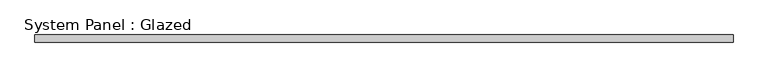
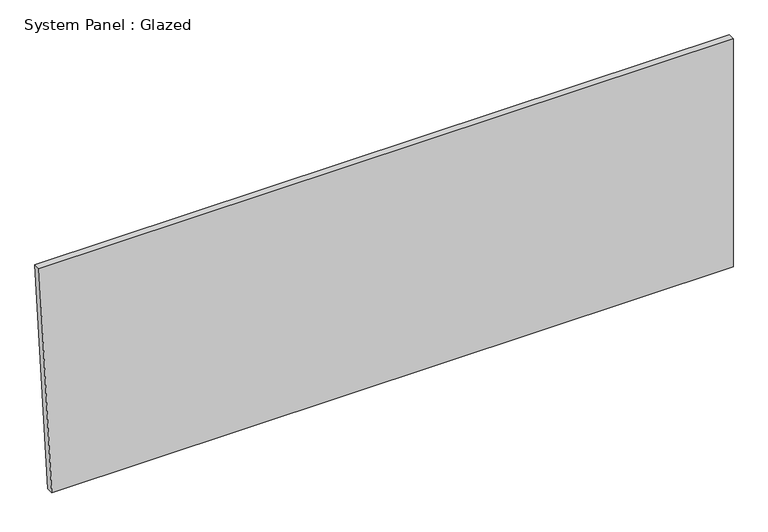
"""IFC4 building model written with IfcOpenShell, lengths in millimetres: plate geometry, System Panel : Glazed."""

import ifcopenshell
import ifcopenshell.guid

model = None  # the IFC model being written
_history = None  # IfcOwnerHistory: only IFC2X3 demands one
_inside = {}  # id of a spatial element -> (the spatial element, [elements in it])
_under = {}  # id of a project, library or spatial element -> (it, [spatial elements below it])
_declared = {}  # id of a project -> (the project, [libraries it declares])
_typed = {}  # id of a type object -> (the type object, [elements of that type])
_made_of = {}  # id of a material, layer set ... -> (it, [elements and type objects made of it])


def new_model(schema):
    """Start an empty IFC model of exactly this schema.

    Asked for "IFC4X3", IfcOpenShell would pick the latest addendum, in which some entities
    have other attributes; the version numbers below select the first issue.
    IFC2X3 requires an IfcOwnerHistory on every rooted entity: one is made here for all.
    """
    global model, _history
    if schema == "IFC4X3":
        model = ifcopenshell.file(schema_version=(4, 3, 0, 0))
    else:
        model = ifcopenshell.file(schema=schema)
    _inside.clear()
    _under.clear()
    _declared.clear()
    _typed.clear()
    _made_of.clear()
    _history = None
    if model.schema == "IFC2X3":
        org = make("IfcOrganization", Name="unknown")
        user = make(
            "IfcPersonAndOrganization",
            ThePerson=make("IfcPerson", FamilyName="unknown"),
            TheOrganization=org,
        )
        app = make(
            "IfcApplication",
            ApplicationDeveloper=org,
            Version="unknown",
            ApplicationFullName="unknown",
            ApplicationIdentifier="unknown",
        )
        _history = make(
            "IfcOwnerHistory",
            OwningUser=user,
            OwningApplication=app,
            ChangeAction="ADDED",
            CreationDate=0,
        )
    return model


def make(cls, **values):
    """One entity of the class cls with the attributes given. An attribute that is None is left unset."""
    return model.create_entity(
        cls, **{name: value for name, value in values.items() if value is not None}
    )


def rooted(cls, **values):
    """An entity with a GlobalId (a new one), such as an element, a storey or a relation."""
    return make(cls, GlobalId=ifcopenshell.guid.new(), OwnerHistory=_history, **values)


def si_unit(unit_type, name, prefix=None):
    """IfcSIUnit, for example si_unit("LENGTHUNIT", "METRE", prefix="MILLI")."""
    return make("IfcSIUnit", UnitType=unit_type, Prefix=prefix, Name=name)


def assignment(units):
    """IfcUnitAssignment: the units of a project."""
    return None if units is None else make("IfcUnitAssignment", Units=units)


def point(xyz):
    """IfcCartesianPoint."""
    return None if xyz is None else make("IfcCartesianPoint", Coordinates=xyz)


def direction(xyz):
    """IfcDirection."""
    return None if xyz is None else make("IfcDirection", DirectionRatios=xyz)


def frame(location, z_axis=None, x_axis=None):
    """IfcAxis2Placement3D, a coordinate frame: its origin and axes. An axis left out is left unset."""
    return make(
        "IfcAxis2Placement3D",
        Location=point(location),
        Axis=direction(z_axis),
        RefDirection=direction(x_axis),
    )


def origin():
    """The frame at (0, 0, 0) with its axes left unset."""
    return frame((0.0, 0.0, 0.0))


def place(relative_to, where):
    """IfcLocalPlacement: puts the frame where relative to a parent placement (None: the world)."""
    return make(
        "IfcLocalPlacement", PlacementRelTo=relative_to, RelativePlacement=where
    )


def context(
    kind, dimensions, precision=None, world=None, true_north=None, identifier=None
):
    """IfcGeometricRepresentationContext, for example the 3D "Model" context."""
    return make(
        "IfcGeometricRepresentationContext",
        ContextIdentifier=identifier,
        ContextType=kind,
        CoordinateSpaceDimension=dimensions,
        Precision=precision,
        WorldCoordinateSystem=world,
        TrueNorth=true_north,
    )


def project(units=None, contexts=None):
    """IfcProject with its units and contexts."""
    return rooted(
        "IfcProject",
        Name="project",
        RepresentationContexts=contexts,
        UnitsInContext=assignment(units),
    )


def spatial(cls, under=None, at=None, **own):
    """A site, building, storey or space (cls), placed at a placement, below another one or the project."""
    s = rooted(cls, ObjectPlacement=at, **own)
    if under is not None:
        _under.setdefault(under.id(), (under, []))[1].append(s)
    return s


def polyline(points):
    """IfcPolyline through the points."""
    return make("IfcPolyline", Points=[point(p) for p in points])


def outline(outer, holes=None, kind="AREA"):
    """IfcArbitraryClosedProfileDef: a profile drawn as a closed curve; with holes, ...WithVoids."""
    if holes is None:
        return make("IfcArbitraryClosedProfileDef", ProfileType=kind, OuterCurve=outer)
    return make(
        "IfcArbitraryProfileDefWithVoids",
        ProfileType=kind,
        OuterCurve=outer,
        InnerCurves=holes,
    )


def extrude(swept, where, along, depth):
    """IfcExtrudedAreaSolid: the profile swept, set in the frame where, extruded along a direction by depth."""
    return make(
        "IfcExtrudedAreaSolid",
        SweptArea=swept,
        Position=where,
        ExtrudedDirection=direction(along),
        Depth=depth,
    )


def shape(context_of_items, identifier, shape_type, items):
    """IfcShapeRepresentation: the items that make up one representation, for example the "Body"."""
    return make(
        "IfcShapeRepresentation",
        ContextOfItems=context_of_items,
        RepresentationIdentifier=identifier,
        RepresentationType=shape_type,
        Items=items,
    )


def source(mapping_origin, context_of_items, identifier, shape_type, items):
    """IfcRepresentationMap: a shape defined once, which mapped items show again and again."""
    return make(
        "IfcRepresentationMap",
        MappingOrigin=mapping_origin,
        MappedRepresentation=shape(context_of_items, identifier, shape_type, items),
    )


def transform(
    local_origin,
    x_axis=None,
    y_axis=None,
    z_axis=None,
    scale=None,
    scale2=None,
    scale3=None,
    uniform=True,
):
    """IfcCartesianTransformationOperator3D, or its non-uniform kind. x_axis, y_axis, z_axis: its Axis1, 2, 3."""
    if uniform:
        return make(
            "IfcCartesianTransformationOperator3D",
            Axis1=direction(x_axis),
            Axis2=direction(y_axis),
            LocalOrigin=point(local_origin),
            Scale=scale,
            Axis3=direction(z_axis),
        )
    return make(
        "IfcCartesianTransformationOperator3DnonUniform",
        Axis1=direction(x_axis),
        Axis2=direction(y_axis),
        LocalOrigin=point(local_origin),
        Scale=scale,
        Axis3=direction(z_axis),
        Scale2=scale2,
        Scale3=scale3,
    )


def mapped(mapping_source, mapping_target):
    """IfcMappedItem: shows the shape of a source again, moved by a transform."""
    return make(
        "IfcMappedItem", MappingSource=mapping_source, MappingTarget=mapping_target
    )


def made_of(thing, what):
    """Note that an element or type object is made of a material, layer set ...; save() writes the relation."""
    if what is not None:
        _made_of.setdefault(what.id(), (what, []))[1].append(thing)
    return thing


def element(
    cls,
    number,
    at=None,
    inside=None,
    cuts=None,
    type_object=None,
    material=None,
    context=None,
    identifier="Body",
    shape_type=None,
    held_by="IfcProductDefinitionShape",
    body=None,
    shapes=None,
    **own,
):
    """One element of the class cls, such as IfcWall. Its Tag is "e" and its number.

    at: its placement. inside: the storey or other place that contains it. cuts: it is an
    opening in that element (IfcRelVoidsElement). A single representation is given by context,
    identifier, shape_type and body (its items); several are given by shapes. held_by: the class
    of the entity that holds the representations. save() writes the other relations.
    """
    e = rooted(cls, Tag="e%d" % number, ObjectPlacement=at, **own)
    if body is not None:
        shapes = [shape(context, identifier, shape_type, body)]
    if shapes is not None:
        e.Representation = make(held_by, Representations=shapes)
    if inside is not None:
        _inside.setdefault(inside.id(), (inside, []))[1].append(e)
    if cuts is not None:
        rooted(
            "IfcRelVoidsElement", RelatingBuildingElement=cuts, RelatedOpeningElement=e
        )
    if type_object is not None:
        _typed.setdefault(type_object.id(), (type_object, []))[1].append(e)
    return made_of(e, material)


def aggregate(whole, parts):
    """IfcRelAggregates: a whole, such as a stair, and the parts it consists of."""
    return rooted("IfcRelAggregates", RelatingObject=whole, RelatedObjects=parts)


def save(model, path):
    """Write the relations noted so far, then the file.

    IfcRelAggregates (storeys below a building ...), IfcRelContainedInSpatialStructure (elements
    in a storey), IfcRelDefinesByType, IfcRelAssociatesMaterial and IfcRelDeclares: one each for
    every whole, place, type object, material and project.
    """
    for whole, parts in _under.values():
        aggregate(whole, parts)
    for where, things in _inside.values():
        rooted(
            "IfcRelContainedInSpatialStructure",
            RelatedElements=things,
            RelatingStructure=where,
        )
    for kind, things in _typed.values():
        rooted("IfcRelDefinesByType", RelatedObjects=things, RelatingType=kind)
    for what, things in _made_of.values():
        rooted("IfcRelAssociatesMaterial", RelatedObjects=things, RelatingMaterial=what)
    for by, libraries in _declared.values():
        rooted("IfcRelDeclares", RelatingContext=by, RelatedDefinitions=libraries)
    model.write(path)


def system_panel_glazed_1dbcaf42(model_context):
    return source(origin(), model_context, "Body", "SweptSolid", [
        extrude(outline(polyline([(0.0, -1202.0248119), (0.0, 1247.3520184), (866.081558, 1247.3520184), (866.081558, -1247.3520184), (0.0, -1202.0248119)])), frame((0.0, -44.45, 0.0), z_axis=(0.0, 1.0, 0.0), x_axis=(0.0, 0.0, 1.0)), (0.0, 0.0, 1.0), 25.4),
    ])


if __name__ == "__main__":
    model = new_model("IFC4")
    model_context = context("Model", 3, world=origin())
    ifc_project = project(units=[si_unit("LENGTHUNIT", "METRE", prefix="MILLI")], contexts=[model_context])
    site = spatial("IfcSite", under=ifc_project)
    building = spatial("IfcBuilding", under=site)
    placement = place(None, origin())
    system_panel_glazed_shape = system_panel_glazed_1dbcaf42(model_context)
    element("IfcPlate", 1, ObjectType="System Panel : Glazed", at=placement, inside=building, context=model_context, shape_type="MappedRepresentation", body=[
        mapped(system_panel_glazed_shape, transform((0.0, 0.0, 0.0), x_axis=(1.0, 0.0, 0.0), y_axis=(0.0, 1.0, 0.0), z_axis=(0.0, 0.0, 1.0))),
    ])
    save(model, "model.ifc")

# Revit data of these elements
# Type "System Panel : Glazed"
#   Construction Type Id = "GSP4R"
#   Analytic Construction = "1/8 in Pilkington single glazing"
#   Visual Light Transmittance = 0.9
#   Solar Heat Gain Coefficient = 0.86
#   Heat Transfer Coefficient (U) = 1.18115 BTU/(h·ft²·°F)
#   Define Thermal Properties by = 1
# Element 1 (IfcPlate, "System Panel : Glazed")
#   Materials on its faces: "Glass"
# Materials
#   "Glass": class "Glass", colour RGB 0 128 192, transparency 0.75, Description = "Soda Lime Glass", Cost = 0
